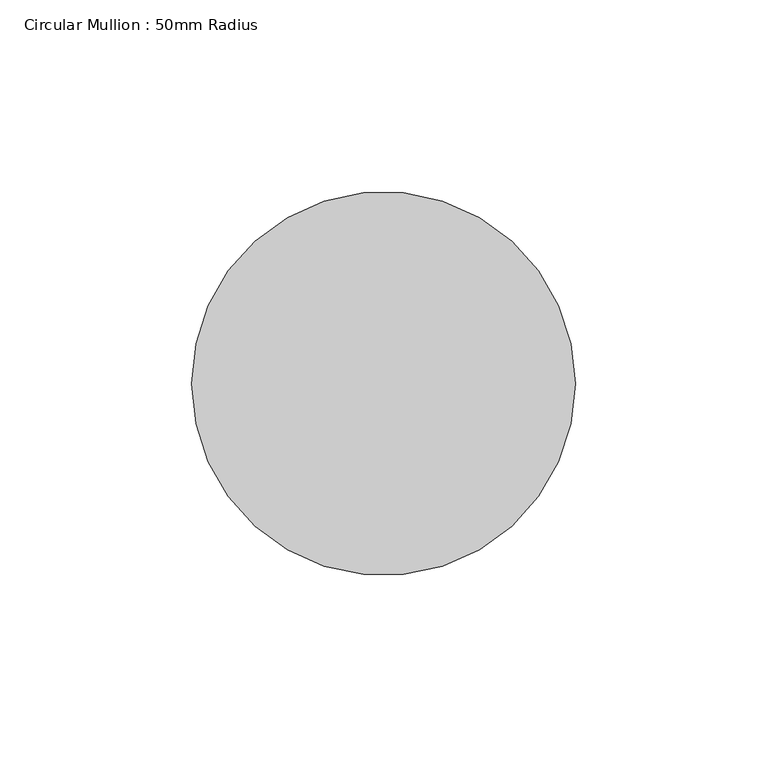
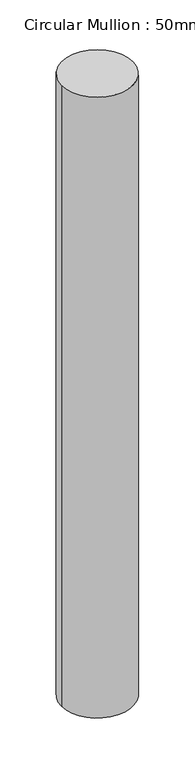
"""IFC4 building model written with IfcOpenShell, lengths in millimetres: member geometry, Circular Mullion : 50mm Radius."""

from ifc_helpers import new_model, si_unit, point, frame, origin, origin_2d, place, context, project, spatial, circle_curve, trimmed, segment, composite_curve, outline, extrude, source, transform, mapped, element, save


def circular_mullion_50mm_radius_63b3a96c(model_context):
    return source(origin(), model_context, "Body", "SweptSolid", [
        extrude(outline(composite_curve([segment(trimmed(circle_curve(origin_2d(), 50.0), [point((50.0, 0.0))], [point((-50.0, 0.0))], False, "CARTESIAN"), True, "CONTINUOUS"), segment(trimmed(circle_curve(origin_2d(), 50.0), [point((-50.0, 0.0))], [point((50.0, 0.0))], False, "CARTESIAN"), True, "CONTINUOUS")], self_intersect=False)), frame((0.0, 0.0, -919.7931749), z_axis=(0.0, 0.0, 1.0), x_axis=(1.0, 0.0, 0.0)), (0.0, 0.0, 1.0), 919.7931749),
    ])


if __name__ == "__main__":
    model = new_model("IFC4")
    model_context = context("Model", 3, world=origin())
    ifc_project = project(units=[si_unit("LENGTHUNIT", "METRE", prefix="MILLI")], contexts=[model_context])
    site = spatial("IfcSite", under=ifc_project)
    building = spatial("IfcBuilding", under=site)
    placement = place(None, origin())
    circular_mullion_50mm_radius_shape = circular_mullion_50mm_radius_63b3a96c(model_context)
    element("IfcMember", 1, ObjectType="Circular Mullion : 50mm Radius", at=placement, inside=building, context=model_context, shape_type="MappedRepresentation", body=[
        mapped(circular_mullion_50mm_radius_shape, transform((0.0, 0.0, 0.0), x_axis=(1.0, 0.0, 0.0), y_axis=(0.0, 1.0, 0.0), z_axis=(0.0, 0.0, 1.0))),
    ])
    save(model, "model.ifc")

# Revit data of these elements
# Type "Circular Mullion : 50mm Radius"
#   built-in parameter 1007350 = 0.164042 (stored number, unit not read)
# Element 1 (IfcMember, "Circular Mullion : 50mm Radius")
#   Materials on its faces: "Aluminium"
# Materials
#   "Aluminium": class "Metal", colour RGB 247 247 247, transparency 0, Description = "Aluminium 6061", Cost = 0
